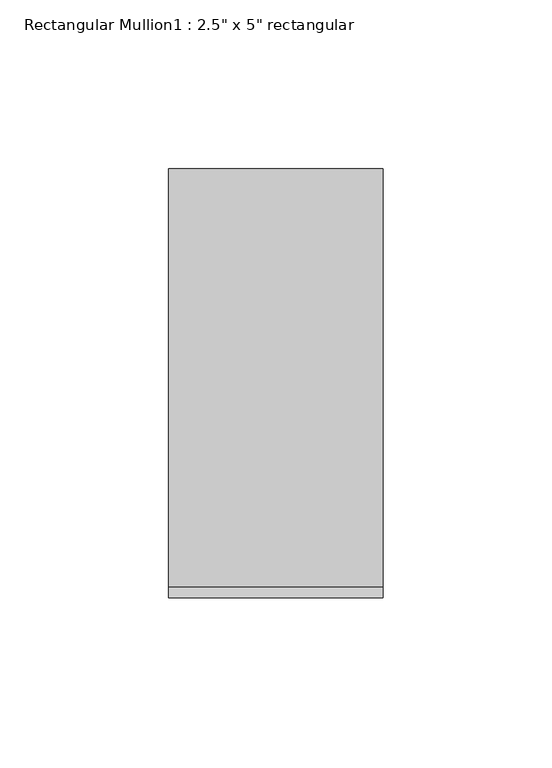
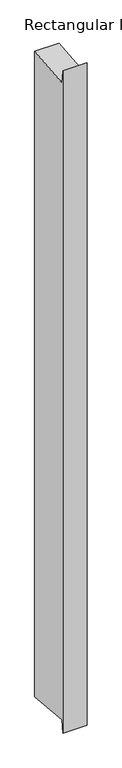
"""IFC4 building model written with IfcOpenShell, lengths in millimetres: member geometry."""

import ifcopenshell
import ifcopenshell.guid

model = None  # the IFC model being written
_history = None  # IfcOwnerHistory: only IFC2X3 demands one
_inside = {}  # id of a spatial element -> (the spatial element, [elements in it])
_under = {}  # id of a project, library or spatial element -> (it, [spatial elements below it])
_declared = {}  # id of a project -> (the project, [libraries it declares])
_typed = {}  # id of a type object -> (the type object, [elements of that type])
_made_of = {}  # id of a material, layer set ... -> (it, [elements and type objects made of it])


def new_model(schema):
    """Start an empty IFC model of exactly this schema.

    Asked for "IFC4X3", IfcOpenShell would pick the latest addendum, in which some entities
    have other attributes; the version numbers below select the first issue.
    IFC2X3 requires an IfcOwnerHistory on every rooted entity: one is made here for all.
    """
    global model, _history
    if schema == "IFC4X3":
        model = ifcopenshell.file(schema_version=(4, 3, 0, 0))
    else:
        model = ifcopenshell.file(schema=schema)
    _inside.clear()
    _under.clear()
    _declared.clear()
    _typed.clear()
    _made_of.clear()
    _history = None
    if model.schema == "IFC2X3":
        org = make("IfcOrganization", Name="unknown")
        user = make(
            "IfcPersonAndOrganization",
            ThePerson=make("IfcPerson", FamilyName="unknown"),
            TheOrganization=org,
        )
        app = make(
            "IfcApplication",
            ApplicationDeveloper=org,
            Version="unknown",
            ApplicationFullName="unknown",
            ApplicationIdentifier="unknown",
        )
        _history = make(
            "IfcOwnerHistory",
            OwningUser=user,
            OwningApplication=app,
            ChangeAction="ADDED",
            CreationDate=0,
        )
    return model


def make(cls, **values):
    """One entity of the class cls with the attributes given. An attribute that is None is left unset."""
    return model.create_entity(
        cls, **{name: value for name, value in values.items() if value is not None}
    )


def rooted(cls, **values):
    """An entity with a GlobalId (a new one), such as an element, a storey or a relation."""
    return make(cls, GlobalId=ifcopenshell.guid.new(), OwnerHistory=_history, **values)


def si_unit(unit_type, name, prefix=None):
    """IfcSIUnit, for example si_unit("LENGTHUNIT", "METRE", prefix="MILLI")."""
    return make("IfcSIUnit", UnitType=unit_type, Prefix=prefix, Name=name)


def assignment(units):
    """IfcUnitAssignment: the units of a project."""
    return None if units is None else make("IfcUnitAssignment", Units=units)


def point(xyz):
    """IfcCartesianPoint."""
    return None if xyz is None else make("IfcCartesianPoint", Coordinates=xyz)


def direction(xyz):
    """IfcDirection."""
    return None if xyz is None else make("IfcDirection", DirectionRatios=xyz)


def frame(location, z_axis=None, x_axis=None):
    """IfcAxis2Placement3D, a coordinate frame: its origin and axes. An axis left out is left unset."""
    return make(
        "IfcAxis2Placement3D",
        Location=point(location),
        Axis=direction(z_axis),
        RefDirection=direction(x_axis),
    )


def origin():
    """The frame at (0, 0, 0) with its axes left unset."""
    return frame((0.0, 0.0, 0.0))


def place(relative_to, where):
    """IfcLocalPlacement: puts the frame where relative to a parent placement (None: the world)."""
    return make(
        "IfcLocalPlacement", PlacementRelTo=relative_to, RelativePlacement=where
    )


def context(
    kind, dimensions, precision=None, world=None, true_north=None, identifier=None
):
    """IfcGeometricRepresentationContext, for example the 3D "Model" context."""
    return make(
        "IfcGeometricRepresentationContext",
        ContextIdentifier=identifier,
        ContextType=kind,
        CoordinateSpaceDimension=dimensions,
        Precision=precision,
        WorldCoordinateSystem=world,
        TrueNorth=true_north,
    )


def project(units=None, contexts=None):
    """IfcProject with its units and contexts."""
    return rooted(
        "IfcProject",
        Name="project",
        RepresentationContexts=contexts,
        UnitsInContext=assignment(units),
    )


def spatial(cls, under=None, at=None, **own):
    """A site, building, storey or space (cls), placed at a placement, below another one or the project."""
    s = rooted(cls, ObjectPlacement=at, **own)
    if under is not None:
        _under.setdefault(under.id(), (under, []))[1].append(s)
    return s


def polyline(points):
    """IfcPolyline through the points."""
    return make("IfcPolyline", Points=[point(p) for p in points])


def outline(outer, holes=None, kind="AREA"):
    """IfcArbitraryClosedProfileDef: a profile drawn as a closed curve; with holes, ...WithVoids."""
    if holes is None:
        return make("IfcArbitraryClosedProfileDef", ProfileType=kind, OuterCurve=outer)
    return make(
        "IfcArbitraryProfileDefWithVoids",
        ProfileType=kind,
        OuterCurve=outer,
        InnerCurves=holes,
    )


def extrude(swept, where, along, depth):
    """IfcExtrudedAreaSolid: the profile swept, set in the frame where, extruded along a direction by depth."""
    return make(
        "IfcExtrudedAreaSolid",
        SweptArea=swept,
        Position=where,
        ExtrudedDirection=direction(along),
        Depth=depth,
    )


def shape(context_of_items, identifier, shape_type, items):
    """IfcShapeRepresentation: the items that make up one representation, for example the "Body"."""
    return make(
        "IfcShapeRepresentation",
        ContextOfItems=context_of_items,
        RepresentationIdentifier=identifier,
        RepresentationType=shape_type,
        Items=items,
    )


def source(mapping_origin, context_of_items, identifier, shape_type, items):
    """IfcRepresentationMap: a shape defined once, which mapped items show again and again."""
    return make(
        "IfcRepresentationMap",
        MappingOrigin=mapping_origin,
        MappedRepresentation=shape(context_of_items, identifier, shape_type, items),
    )


def transform(
    local_origin,
    x_axis=None,
    y_axis=None,
    z_axis=None,
    scale=None,
    scale2=None,
    scale3=None,
    uniform=True,
):
    """IfcCartesianTransformationOperator3D, or its non-uniform kind. x_axis, y_axis, z_axis: its Axis1, 2, 3."""
    if uniform:
        return make(
            "IfcCartesianTransformationOperator3D",
            Axis1=direction(x_axis),
            Axis2=direction(y_axis),
            LocalOrigin=point(local_origin),
            Scale=scale,
            Axis3=direction(z_axis),
        )
    return make(
        "IfcCartesianTransformationOperator3DnonUniform",
        Axis1=direction(x_axis),
        Axis2=direction(y_axis),
        LocalOrigin=point(local_origin),
        Scale=scale,
        Axis3=direction(z_axis),
        Scale2=scale2,
        Scale3=scale3,
    )


def mapped(mapping_source, mapping_target):
    """IfcMappedItem: shows the shape of a source again, moved by a transform."""
    return make(
        "IfcMappedItem", MappingSource=mapping_source, MappingTarget=mapping_target
    )


def made_of(thing, what):
    """Note that an element or type object is made of a material, layer set ...; save() writes the relation."""
    if what is not None:
        _made_of.setdefault(what.id(), (what, []))[1].append(thing)
    return thing


def element(
    cls,
    number,
    at=None,
    inside=None,
    cuts=None,
    type_object=None,
    material=None,
    context=None,
    identifier="Body",
    shape_type=None,
    held_by="IfcProductDefinitionShape",
    body=None,
    shapes=None,
    **own,
):
    """One element of the class cls, such as IfcWall. Its Tag is "e" and its number.

    at: its placement. inside: the storey or other place that contains it. cuts: it is an
    opening in that element (IfcRelVoidsElement). A single representation is given by context,
    identifier, shape_type and body (its items); several are given by shapes. held_by: the class
    of the entity that holds the representations. save() writes the other relations.
    """
    e = rooted(cls, Tag="e%d" % number, ObjectPlacement=at, **own)
    if body is not None:
        shapes = [shape(context, identifier, shape_type, body)]
    if shapes is not None:
        e.Representation = make(held_by, Representations=shapes)
    if inside is not None:
        _inside.setdefault(inside.id(), (inside, []))[1].append(e)
    if cuts is not None:
        rooted(
            "IfcRelVoidsElement", RelatingBuildingElement=cuts, RelatedOpeningElement=e
        )
    if type_object is not None:
        _typed.setdefault(type_object.id(), (type_object, []))[1].append(e)
    return made_of(e, material)


def aggregate(whole, parts):
    """IfcRelAggregates: a whole, such as a stair, and the parts it consists of."""
    return rooted("IfcRelAggregates", RelatingObject=whole, RelatedObjects=parts)


def save(model, path):
    """Write the relations noted so far, then the file.

    IfcRelAggregates (storeys below a building ...), IfcRelContainedInSpatialStructure (elements
    in a storey), IfcRelDefinesByType, IfcRelAssociatesMaterial and IfcRelDeclares: one each for
    every whole, place, type object, material and project.
    """
    for whole, parts in _under.values():
        aggregate(whole, parts)
    for where, things in _inside.values():
        rooted(
            "IfcRelContainedInSpatialStructure",
            RelatedElements=things,
            RelatingStructure=where,
        )
    for kind, things in _typed.values():
        rooted("IfcRelDefinesByType", RelatedObjects=things, RelatingType=kind)
    for what, things in _made_of.values():
        rooted("IfcRelAssociatesMaterial", RelatedObjects=things, RelatingMaterial=what)
    for by, libraries in _declared.values():
        rooted("IfcRelDeclares", RelatingContext=by, RelatedDefinitions=libraries)
    model.write(path)


def member_b9454cfc(model_context):
    return source(origin(), model_context, "Body", "SweptSolid", [
        extrude(outline(polyline([(-63.5, 28.7582862), (-60.2336356, -5.8295375), (63.5, 5.8554746), (63.5, -1771.1554746), (-60.2336356, -1759.4704625), (-63.5, -1794.0582862), (-63.5, 28.7582862)])), frame((-63.5, 0.0, 0.0), z_axis=(1.0, 0.0, 0.0), x_axis=(0.0, 1.0, 0.0)), (0.0, 0.0, 1.0), 63.5),
    ])


if __name__ == "__main__":
    model = new_model("IFC4")
    model_context = context("Model", 3, world=origin())
    ifc_project = project(units=[si_unit("LENGTHUNIT", "METRE", prefix="MILLI")], contexts=[model_context])
    site = spatial("IfcSite", under=ifc_project)
    building = spatial("IfcBuilding", under=site)
    placement = place(None, origin())
    member_shape = member_b9454cfc(model_context)
    element("IfcMember", 1, ObjectType="Rectangular Mullion1 : 2.5\" x 5\" rectangular", at=placement, inside=building, context=model_context, shape_type="MappedRepresentation", body=[
        mapped(member_shape, transform((0.0, 0.0, 0.0), x_axis=(1.0, 0.0, 0.0), y_axis=(0.0, 1.0, 0.0), z_axis=(0.0, 0.0, 1.0))),
    ])
    save(model, "model.ifc")

# Revit data of these elements
# Type "Rectangular Mullion1 : 2.5\" x 5\" rectangular"
#   built-in parameter 1007304 = 0.416667 (stored number, unit not read)
#   built-in parameter 1007301 = 0.104167 (stored number, unit not read)
#   built-in parameter 1007300 = 0.104167 (stored number, unit not read)
# Element 1 (IfcMember, "Rectangular Mullion1 : 2.5\" x 5\" rectangular")
#   Materials on its faces: "support-frame"
# Materials
#   "support-frame": class "Unassigned", colour RGB 233 233 233, transparency 0, Cost = 0
